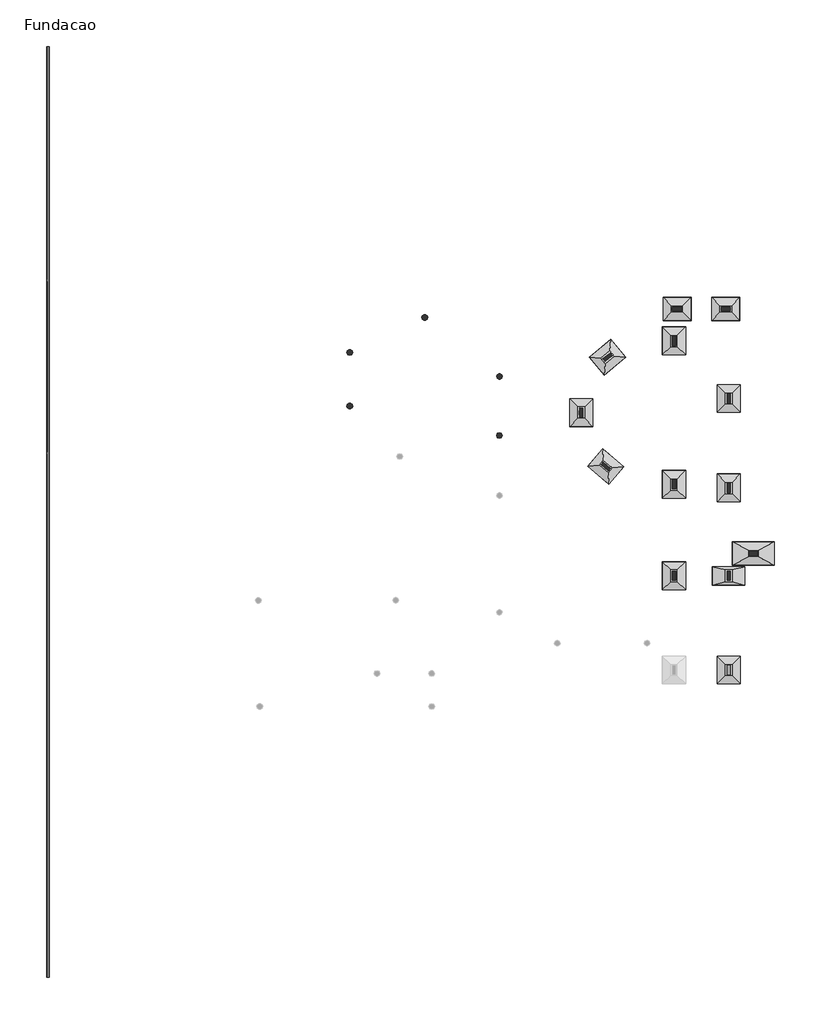
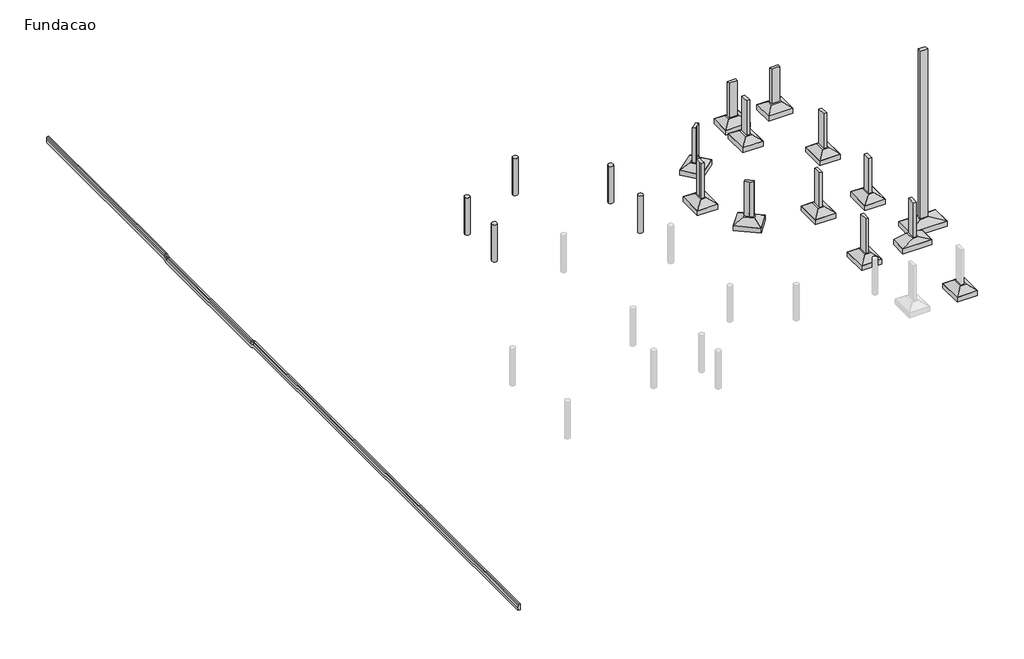
# One storey, part 2 of 2: 17 columns, 13 fasteners, 1 proxy.
# Revit data of these elements (continued)
# Element 3 (IfcColumn, "TQS - Pilar circular : TQS - Pilar circular 25.0cm") (continued)
#   Concreto C = ""
#   Taxa de armadura (kgf/m³) = 0
#   Carga (tf/m²) = 0
#   Carga (tf/m) = 0
#   Carga (tf) = 0
#   Altura = 1.70 m
#   Rebaixo = 0.00 m
#   Altura da fundacao = 0.00 m
#   Largura = 0.00 m
#   Distancia a face = 0.00 m
#   Distancia ao eixo = 0.00 m
#   Resultado de Ensaios fck (MPa) = 0
#   Unique TQS ID = -767
#   Principal = yes
#   Nasce = yes
#   Morre = yes
#   Cabeca de Pilar = no
#   Structural Material = Concrete - Cast-in-Place Concrete
#   Phase Created = CC_AP/ESTR
#   Materials on its faces: "Concrete - Cast-in-Place Concrete"
# Element 4 (IfcColumn, "TQS - Pilar circular : TQS - Pilar circular 25.0cm")
#   Uso = "ESTRUTURA"
#   Titulo = "B3"
#   Chave = "B3//0"
#   Tipo Elemento = "Pilar"
#   SHA1 = "B4824BA6EB04DBA88013BAD919A11F987E93A8CE"
#   Revisão = ""
#   Tipo de carga = ""
#   Divisor de flexao = ""
#   Secao = "C 25"
#   Configuracao = ""
#   Angulo (graus) = ""
#   Detalhamento = ""
#   Casos de vento manual = ""
#   Tipo = ""
#   Alcas = ""
#   Furos = ""
#   Pino = ""
#   Distribuicao = ""
#   Solidarizado = ""
#   Solidarizar na montagem = ""
#   Unir com o próximo = ""
#   Grupo pre moldado = ""
#   Verificado = ""
#   Concreto C = ""
#   Taxa de armadura (kgf/m³) = 0
#   Carga (tf/m²) = 0
#   Carga (tf/m) = 0
#   Carga (tf) = 0
#   Altura = 1.70 m
#   Rebaixo = 0.00 m
#   Altura da fundacao = 0.00 m
#   Largura = 0.00 m
#   Distancia a face = 0.00 m
#   Distancia ao eixo = 0.00 m
#   Resultado de Ensaios fck (MPa) = 0
#   Unique TQS ID = -768
#   Principal = yes
#   Nasce = yes
#   Morre = yes
#   Cabeca de Pilar = no
#   Structural Material = Concrete - Cast-in-Place Concrete
#   Phase Created = CC_AP/ESTR
#   Materials on its faces: "Concrete - Cast-in-Place Concrete"
# Element 5 (IfcColumn, "TQS - Pilar circular : TQS - Pilar circular 25.0cm")
#   Uso = "ESTRUTURA"
#   Titulo = "B2"
#   Chave = "B2//0"
#   Tipo Elemento = "Pilar"
#   SHA1 = "4CE2E912DC9B0318D735B89447CA6954BE93FBBD"
#   Revisão = ""
#   Tipo de carga = ""
#   Divisor de flexao = ""
#   Secao = "C 25"
#   Configuracao = ""
#   Angulo (graus) = ""
#   Detalhamento = ""
#   Casos de vento manual = ""
#   Tipo = ""
#   Alcas = ""
#   Furos = ""
#   Pino = ""
#   Distribuicao = ""
#   Solidarizado = ""
#   Solidarizar na montagem = ""
#   Unir com o próximo = ""
#   Grupo pre moldado = ""
#   Verificado = ""
#   Concreto C = ""
#   Taxa de armadura (kgf/m³) = 0
#   Carga (tf/m²) = 0
#   Carga (tf/m) = 0
#   Carga (tf) = 0
#   Altura = 1.70 m
#   Rebaixo = 0.00 m
#   Altura da fundacao = 0.00 m
#   Largura = 0.00 m
#   Distancia a face = 0.00 m
#   Distancia ao eixo = 0.00 m
#   Resultado de Ensaios fck (MPa) = 0
#   Unique TQS ID = -773
#   Principal = yes
#   Nasce = yes
#   Morre = yes
#   Cabeca de Pilar = no
#   Structural Material = Concrete - Cast-in-Place Concrete
#   Phase Created = CC_AP/ESTR
#   Materials on its faces: "Concrete - Cast-in-Place Concrete"
# Element 6 (IfcColumn, "TQS - Pilar circular : TQS - Pilar circular 25.0cm")
#   Uso = "ESTRUTURA"
#   Titulo = "B4"
#   Chave = "B4//0"
#   Tipo Elemento = "Pilar"
#   SHA1 = "33C063B82A35DA14032FDD3FDBBCC7600ACCE04D"
#   Revisão = ""
#   Tipo de carga = ""
#   Divisor de flexao = ""
#   Secao = "C 25"
#   Configuracao = ""
#   Angulo (graus) = ""
#   Detalhamento = ""
#   Casos de vento manual = ""
#   Tipo = ""
#   Alcas = ""
#   Furos = ""
#   Pino = ""
#   Distribuicao = ""
#   Solidarizado = ""
#   Solidarizar na montagem = ""
#   Unir com o próximo = ""
#   Grupo pre moldado = ""
#   Verificado = ""
#   Concreto C = ""
#   Taxa de armadura (kgf/m³) = 0
#   Carga (tf/m²) = 0
#   Carga (tf/m) = 0
#   Carga (tf) = 0
#   Altura = 1.70 m
#   Rebaixo = 0.00 m
#   Altura da fundacao = 0.00 m
#   Largura = 0.00 m
#   Distancia a face = 0.00 m
#   Distancia ao eixo = 0.00 m
#   Resultado de Ensaios fck (MPa) = 0
#   Unique TQS ID = -774
#   Principal = yes
#   Nasce = yes
#   Morre = yes
#   Cabeca de Pilar = no
#   Structural Material = Concrete - Cast-in-Place Concrete
#   Phase Created = CC_AP/ESTR
#   Materials on its faces: "Concrete - Cast-in-Place Concrete"
# Element 7 (IfcColumn, "TQS - Pilar retangular : 14.0 x 40.0")
#   Uso = "ESTRUTURA"
#   Titulo = "PS1"
#   Chave = "PS1//0"
#   Tipo Elemento = "Pilar"
#   SHA1 = "4597F8CE5B5008DD3216867DEF2D1334C590FC15"
#   Revisão = ""
#   Tipo de carga = ""
#   Divisor de flexao = ""
#   Secao = "R 14/40 270°"
#   Configuracao = ""
#   Angulo (graus) = ""
#   Detalhamento = ""
#   Casos de vento manual = ""
#   Tipo = ""
#   Alcas = ""
#   Furos = ""
#   Pino = ""
#   Distribuicao = ""
#   Solidarizado = ""
#   Solidarizar na montagem = ""
#   Unir com o próximo = ""
#   Grupo pre moldado = ""
#   Verificado = ""
#   Concreto C = ""
#   Taxa de armadura (kgf/m³) = 0
#   Carga (tf/m²) = 0
#   Carga (tf/m) = 0
#   Carga (tf) = 0
#   Altura = 1.70 m
#   Rebaixo = 0.00 m
#   Altura da fundacao = 0.00 m
#   Largura = 0.00 m
#   Distancia a face = 0.00 m
#   Distancia ao eixo = 0.00 m
#   Resultado de Ensaios fck (MPa) = 0
#   Unique TQS ID = -958
#   Principal = yes
#   Nasce = yes
#   Morre = yes
#   Cabeca de Pilar = no
#   Structural Material = Concrete - Cast-in-Place Concrete
#   Phase Created = CC_AP/ESTR
#   Materials on its faces: "Concrete - Cast-in-Place Concrete"
# Element 8 (IfcColumn, "TQS - Pilar retangular : 14.0 x 40.0")
#   Uso = "ESTRUTURA"
#   Titulo = "PS2"
#   Chave = "PS2//0"
#   Tipo Elemento = "Pilar"
#   SHA1 = "1729CD9DA72122FACD843418D908847D3B1966CD"
#   Revisão = ""
#   Tipo de carga = ""
#   Divisor de flexao = ""
#   Secao = "R 14/40 270°"
#   Configuracao = ""
#   Angulo (graus) = ""
#   Detalhamento = ""
#   Casos de vento manual = ""
#   Tipo = ""
#   Alcas = ""
#   Furos = ""
#   Pino = ""
#   Distribuicao = ""
#   Solidarizado = ""
#   Solidarizar na montagem = ""
#   Unir com o próximo = ""
#   Grupo pre moldado = ""
#   Verificado = ""
#   Concreto C = ""
#   Taxa de armadura (kgf/m³) = 0
#   Carga (tf/m²) = 0
#   Carga (tf/m) = 0
#   Carga (tf) = 0
#   Altura = 1.70 m
#   Rebaixo = 0.00 m
#   Altura da fundacao = 0.00 m
#   Largura = 0.00 m
#   Distancia a face = 0.00 m
#   Distancia ao eixo = 0.00 m
#   Resultado de Ensaios fck (MPa) = 0
#   Unique TQS ID = -959
#   Principal = yes
#   Nasce = yes
#   Morre = yes
#   Cabeca de Pilar = no
#   Structural Material = Concrete - Cast-in-Place Concrete
#   Phase Created = CC_AP/ESTR
#   Materials on its faces: "Concrete - Cast-in-Place Concrete"
# Element 9 (IfcColumn, "TQS - Pilar retangular : 14.0 x 40.0")
#   Uso = "ESTRUTURA"
#   Titulo = "PS3"
#   Chave = "PS3//0"
#   Tipo Elemento = "Pilar"
#   SHA1 = "E1C4E1DD2B85E2F78CE9D8770BC24705A0EC4463"
#   Revisão = ""
#   Tipo de carga = ""
#   Divisor de flexao = ""
#   Secao = "R 14/40 180°"
#   Configuracao = ""
#   Angulo (graus) = ""
#   Detalhamento = ""
#   Casos de vento manual = ""
#   Tipo = ""
#   Alcas = ""
#   Furos = ""
#   Pino = ""
#   Distribuicao = ""
#   Solidarizado = ""
#   Solidarizar na montagem = ""
#   Unir com o próximo = ""
#   Grupo pre moldado = ""
#   Verificado = ""
#   Concreto C = ""
#   Taxa de armadura (kgf/m³) = 0
#   Carga (tf/m²) = 0
#   Carga (tf/m) = 0
#   Carga (tf) = 0
#   Altura = 1.70 m
#   Rebaixo = 0.00 m
#   Altura da fundacao = 0.00 m
#   Largura = 0.00 m
#   Distancia a face = 0.00 m
#   Distancia ao eixo = 0.00 m
#   Resultado de Ensaios fck (MPa) = 0
#   Unique TQS ID = -960
#   Principal = yes
#   Nasce = yes
#   Morre = yes
#   Cabeca de Pilar = no
#   Structural Material = Concrete - Cast-in-Place Concrete
#   Phase Created = CC_AP/ESTR
#   Materials on its faces: "Concrete - Cast-in-Place Concrete"
# Element 10 (IfcColumn, "TQS - Pilar retangular : 14.0 x 40.0")
#   Uso = "ESTRUTURA"
#   Titulo = "PS7"
#   Chave = "PS7//0"
#   Tipo Elemento = "Pilar"
#   SHA1 = "EE51B7F018C373FE9CEF53A9864C8051348A9FB9"
#   Revisão = ""
#   Tipo de carga = ""
#   Divisor de flexao = ""
#   Secao = "R 14/40 180°"
#   Configuracao = ""
#   Angulo (graus) = ""
#   Detalhamento = ""
#   Casos de vento manual = ""
#   Tipo = ""
#   Alcas = ""
#   Furos = ""
#   Pino = ""
#   Distribuicao = ""
#   Solidarizado = ""
#   Solidarizar na montagem = ""
#   Unir com o próximo = ""
#   Grupo pre moldado = ""
#   Verificado = ""
#   Concreto C = ""
#   Taxa de armadura (kgf/m³) = 0
#   Carga (tf/m²) = 0
#   Carga (tf/m) = 0
#   Carga (tf) = 0
#   Altura = 1.70 m
#   Rebaixo = 0.00 m
#   Altura da fundacao = 0.00 m
#   Largura = 0.00 m
#   Distancia a face = 0.00 m
#   Distancia ao eixo = 0.00 m
#   Resultado de Ensaios fck (MPa) = 0
#   Unique TQS ID = -964
#   Principal = yes
#   Nasce = yes
#   Morre = yes
#   Cabeca de Pilar = no
#   Structural Material = Concrete - Cast-in-Place Concrete
#   Phase Created = CC_AP/ESTR
#   Materials on its faces: "Concrete - Cast-in-Place Concrete"
# Element 11 (IfcColumn, "TQS - Pilar retangular : 14.0 x 40.0")
#   Uso = "ESTRUTURA"
#   Titulo = "PS8"
#   Chave = "PS8//0"
#   Tipo Elemento = "Pilar"
#   SHA1 = "B515A8CC25CBD0A114828B82A1075E16319BC015"
#   Revisão = ""
#   Tipo de carga = ""
#   Divisor de flexao = ""
#   Secao = "R 14/40 180°"
#   Configuracao = ""
#   Angulo (graus) = ""
#   Detalhamento = ""
#   Casos de vento manual = ""
#   Tipo = ""
#   Alcas = ""
#   Furos = ""
#   Pino = ""
#   Distribuicao = ""
#   Solidarizado = ""
#   Solidarizar na montagem = ""
#   Unir com o próximo = ""
#   Grupo pre moldado = ""
#   Verificado = ""
#   Concreto C = ""
#   Taxa de armadura (kgf/m³) = 0
#   Carga (tf/m²) = 0
#   Carga (tf/m) = 0
#   Carga (tf) = 0
#   Altura = 1.70 m
#   Rebaixo = 0.00 m
#   Altura da fundacao = 0.00 m
#   Largura = 0.00 m
#   Distancia a face = 0.00 m
#   Distancia ao eixo = 0.00 m
#   Resultado de Ensaios fck (MPa) = 0
#   Unique TQS ID = -965
#   Principal = yes
#   Nasce = yes
#   Morre = yes
#   Cabeca de Pilar = no
#   Structural Material = Concrete - Cast-in-Place Concrete
#   Phase Created = CC_AP/ESTR
#   Materials on its faces: "Concrete - Cast-in-Place Concrete"
# Element 12 (IfcColumn, "TQS - Pilar retangular : 14.0 x 40.0")
#   Uso = "ESTRUTURA"
#   Titulo = "PS11"
#   Chave = "PS11//0"
#   Tipo Elemento = "Pilar"
#   SHA1 = "38C3E9E25C80C043D595FE86FE1A911FDC38D350"
#   Revisão = ""
#   Tipo de carga = ""
#   Divisor de flexao = ""
#   Secao = "R 14/40 180°"
#   Configuracao = ""
#   Angulo (graus) = ""
#   Detalhamento = ""
#   Casos de vento manual = ""
#   Tipo = ""
#   Alcas = ""
#   Furos = ""
#   Pino = ""
#   Distribuicao = ""
#   Solidarizado = ""
#   Solidarizar na montagem = ""
#   Unir com o próximo = ""
#   Grupo pre moldado = ""
#   Verificado = ""
#   Concreto C = ""
#   Taxa de armadura (kgf/m³) = 0
#   Carga (tf/m²) = 0
#   Carga (tf/m) = 0
#   Carga (tf) = 0
#   Altura = 1.70 m
#   Rebaixo = 0.00 m
#   Altura da fundacao = 0.00 m
#   Largura = 0.00 m
#   Distancia a face = 0.00 m
#   Distancia ao eixo = 0.00 m
#   Resultado de Ensaios fck (MPa) = 0
#   Unique TQS ID = -968
#   Principal = yes
#   Nasce = yes
#   Morre = yes
#   Cabeca de Pilar = no
#   Structural Material = Concrete - Cast-in-Place Concrete
#   Phase Created = CC_AP/ESTR
#   Materials on its faces: "Concrete - Cast-in-Place Concrete"
# Element 13 (IfcColumn, "TQS - Pilar retangular : 14.0 x 40.0")
#   Uso = "ESTRUTURA"
#   Titulo = "PS12"
#   Chave = "PS12//0"
#   Tipo Elemento = "Pilar"
#   SHA1 = "512D0DE7DB718BC0FE0AECE12A9FB23F7FBE26A9"
#   Revisão = ""
#   Tipo de carga = ""
#   Divisor de flexao = ""
#   Secao = "R 14/40 180°"
#   Configuracao = ""
#   Angulo (graus) = ""
#   Detalhamento = ""
#   Casos de vento manual = ""
#   Tipo = ""
#   Alcas = ""
#   Furos = ""
#   Pino = ""
#   Distribuicao = ""
#   Solidarizado = ""
#   Solidarizar na montagem = ""
#   Unir com o próximo = ""
#   Grupo pre moldado = ""
#   Verificado = ""
#   Concreto C = ""
#   Taxa de armadura (kgf/m³) = 0
#   Carga (tf/m²) = 0
#   Carga (tf/m) = 0
#   Carga (tf) = 0
#   Altura = 1.70 m
#   Rebaixo = 0.00 m
#   Altura da fundacao = 0.00 m
#   Largura = 0.00 m
#   Distancia a face = 0.00 m
#   Distancia ao eixo = 0.00 m
#   Resultado de Ensaios fck (MPa) = 0
#   Unique TQS ID = -969
#   Principal = yes
#   Nasce = yes
#   Morre = yes
#   Cabeca de Pilar = no
#   Structural Material = Concrete - Cast-in-Place Concrete
#   Phase Created = CC_AP/ESTR
#   Materials on its faces: "Concrete - Cast-in-Place Concrete"
# Element 14 (IfcColumn, "TQS - Pilar retangular : 14.0 x 40.0")
#   Uso = "ESTRUTURA"
#   Titulo = "PS13"
#   Chave = "PS13//0"
#   Tipo Elemento = "Pilar"
#   SHA1 = "8EC8E2C6B90DD4DF760F1D4ED431316ED84D10F2"
#   Revisão = ""
#   Tipo de carga = ""
#   Divisor de flexao = ""
#   Secao = "R 14/40 180°"
#   Configuracao = ""
#   Angulo (graus) = ""
#   Detalhamento = ""
#   Casos de vento manual = ""
#   Tipo = ""
#   Alcas = ""
#   Furos = ""
#   Pino = ""
#   Distribuicao = ""
#   Solidarizado = ""
#   Solidarizar na montagem = ""
#   Unir com o próximo = ""
#   Grupo pre moldado = ""
#   Verificado = ""
#   Concreto C = ""
#   Taxa de armadura (kgf/m³) = 0
#   Carga (tf/m²) = 0
#   Carga (tf/m) = 0
#   Carga (tf) = 0
#   Altura = 1.70 m
#   Rebaixo = 0.00 m
#   Altura da fundacao = 0.00 m
#   Largura = 0.00 m
#   Distancia a face = 0.00 m
#   Distancia ao eixo = 0.00 m
#   Resultado de Ensaios fck (MPa) = 0
#   Unique TQS ID = -970
#   Principal = yes
#   Nasce = yes
#   Morre = yes
#   Cabeca de Pilar = no
#   Structural Material = Concrete - Cast-in-Place Concrete
#   Phase Created = CC_AP/ESTR
#   Materials on its faces: "Concrete - Cast-in-Place Concrete"
# Element 15 (IfcColumn, "TQS - Pilar retangular : 19.0 x 35.0")
#   Uso = "ESTRUTURA"
#   Titulo = "P14"
#   Chave = "P14//0"
#   Tipo Elemento = "Pilar"
#   SHA1 = "6631C03D899D7914EBA5EACF44BE1498A45C603B"
#   Revisão = ""
#   Tipo de carga = ""
#   Divisor de flexao = ""
#   Secao = "R 19/35 90°"
#   Configuracao = ""
#   Angulo (graus) = ""
#   Detalhamento = ""
#   Casos de vento manual = ""
#   Tipo = ""
#   Alcas = ""
#   Furos = ""
#   Pino = ""
#   Distribuicao = ""
#   Solidarizado = ""
#   Solidarizar na montagem = ""
#   Unir com o próximo = ""
#   Grupo pre moldado = ""
#   Verificado = ""
#   Concreto C = ""
#   Taxa de armadura (kgf/m³) = 0
#   Carga (tf/m²) = 0
#   Carga (tf/m) = 0
#   Carga (tf) = 0
#   Altura = 7.85 m
#   Rebaixo = 0.00 m
#   Altura da fundacao = 0.00 m
#   Largura = 0.00 m
#   Distancia a face = 0.00 m
#   Distancia ao eixo = 0.00 m
#   Resultado de Ensaios fck (MPa) = 0
#   Unique TQS ID = -30
#   Principal = yes
#   Nasce = yes
#   Morre = yes
#   Cabeca de Pilar = no
#   Structural Material = Concrete - Cast-in-Place Concrete
#   Phase Created = CC_AP/ESTR
#   Materials on its faces: "Concrete - Cast-in-Place Concrete"
# Element 16 (IfcColumn, "TQS - Pilar Polig_1 : TQS Column")
#   Uso = "ESTRUTURA"
#   Titulo = "PS4"
#   Chave = "PS4//0"
#   Tipo Elemento = "Pilar"
#   SHA1 = "CAF5758E71A5FE097847EBD6542E0EE23CE53B7B"
#   Revisão = ""
#   Tipo de carga = ""
#   Divisor de flexao = ""
#   Secao = "P  - Poligonal"
#   Configuracao = ""
#   Angulo (graus) = ""
#   Detalhamento = ""
#   Casos de vento manual = ""
#   Tipo = ""
#   Alcas = ""
#   Furos = ""
#   Pino = ""
#   Distribuicao = ""
#   Solidarizado = ""
#   Solidarizar na montagem = ""
#   Unir com o próximo = ""
#   Grupo pre moldado = ""
#   Verificado = ""
#   Concreto C = ""
#   Taxa de armadura (kgf/m³) = 0
#   Carga (tf/m²) = 0
#   Carga (tf/m) = 0
#   Carga (tf) = 0
#   Altura = 1.70 m
#   Rebaixo = 0.00 m
#   Altura da fundacao = 0.00 m
#   Largura = 0.00 m
#   Distancia a face = 0.00 m
#   Distancia ao eixo = 0.00 m
#   Resultado de Ensaios fck (MPa) = 0
#   Unique TQS ID = -961
#   Principal = yes
#   Nasce = yes
#   Morre = yes
#   Cabeca de Pilar = no
#   Structural Material = Concrete - Cast-in-Place Concrete
#   Phase Created = CC_AP/ESTR
# Element 17 (IfcColumn, "TQS - Pilar Polig_1 : TQS Column")
#   Uso = "ESTRUTURA"
#   Titulo = "PS5"
#   Chave = "PS5//0"
#   Tipo Elemento = "Pilar"
#   SHA1 = "AE9BDBDC0B1786B9555B7E0CE4AAD4E849800AD1"
#   Revisão = ""
#   Tipo de carga = ""
#   Divisor de flexao = ""
#   Secao = "P  - Poligonal"
#   Configuracao = ""
#   Angulo (graus) = ""
#   Detalhamento = ""
#   Casos de vento manual = ""
#   Tipo = ""
#   Alcas = ""
#   Furos = ""
#   Pino = ""
#   Distribuicao = ""
#   Solidarizado = ""
#   Solidarizar na montagem = ""
#   Unir com o próximo = ""
#   Grupo pre moldado = ""
#   Verificado = ""
#   Concreto C = ""
#   Taxa de armadura (kgf/m³) = 0
#   Carga (tf/m²) = 0
#   Carga (tf/m) = 0
#   Carga (tf) = 0
#   Altura = 1.70 m
#   Rebaixo = 0.00 m
#   Altura da fundacao = 0.00 m
#   Largura = 0.00 m
#   Distancia a face = 0.00 m
#   Distancia ao eixo = 0.00 m
#   Resultado de Ensaios fck (MPa) = 0
#   Unique TQS ID = -962
#   Principal = yes
#   Nasce = yes
#   Morre = yes
#   Cabeca de Pilar = no
#   Structural Material = Concrete - Cast-in-Place Concrete
#   Phase Created = CC_AP/ESTR
# Element 18 (IfcColumn, "TQS - Pilar Polig_2 : TQS Column")
#   Uso = "ESTRUTURA"
#   Titulo = "PS6"
#   Chave = "PS6//0"
#   Tipo Elemento = "Pilar"
#   SHA1 = "07EEAEB0E5A3D9C7C5812BCB6FDA506A68E4D4F2"
#   Revisão = ""
#   Tipo de carga = ""
#   Divisor de flexao = ""
#   Secao = "P  - Poligonal"
#   Configuracao = ""
#   Angulo (graus) = ""
#   Detalhamento = ""
#   Casos de vento manual = ""
#   Tipo = ""
#   Alcas = ""
#   Furos = ""
#   Pino = ""
#   Distribuicao = ""
#   Solidarizado = ""
#   Solidarizar na montagem = ""
#   Unir com o próximo = ""
#   Grupo pre moldado = ""
#   Verificado = ""
#   Concreto C = ""
#   Taxa de armadura (kgf/m³) = 0
#   Carga (tf/m²) = 0
#   Carga (tf/m) = 0
#   Carga (tf) = 0
#   Altura = 1.70 m
#   Rebaixo = 0.00 m
#   Altura da fundacao = 0.00 m
#   Largura = 0.00 m
#   Distancia a face = 0.00 m
#   Distancia ao eixo = 0.00 m
#   Resultado de Ensaios fck (MPa) = 0
#   Unique TQS ID = -963
#   Principal = yes
#   Nasce = yes
#   Morre = yes
#   Cabeca de Pilar = no
#   Structural Material = Concrete - Cast-in-Place Concrete
#   Phase Created = CC_AP/ESTR
# Element 19 (IfcFastener, "TQS - Sapata : S14")
#   Uso = "ESTRUTURA"
#   Titulo = "S14"
#   Chave = "-1550"
#   Tipo Elemento = "Fundação"
#   SHA1 = "1357E856F80250D7EFC9EC1E050D5963CC884844"
#   Revisão = ""
#   Tipo de carga = ""
#   Divisor de flexao = ""
#   Secao = ""
#   Configuracao = ""
#   Angulo (graus) = ""
#   Detalhamento = ""
#   Casos de vento manual = ""
#   Tipo = "Sapata"
#   Dimensoes = "100.0,180.0"
#   Estacas = ""
#   Calice = ""
#   Rugosidade = ""
#   Alcas = ""
#   Furos = ""
#   Pino = ""
#   Distribuicao = ""
#   Solidarizado = ""
#   Solidarizar na montagem = ""
#   Unir com o próximo = ""
#   Grupo pre moldado = ""
#   Verificado = ""
#   Concreto C = ""
#   Taxa de armadura (kgf/m³) = 0
#   Carga (tf/m²) = 0
#   Carga (tf/m) = 0
#   Carga (tf) = 0
#   Altura = 0.00 m
#   Rebaixo = 0.00 m
#   Pilar ficticio = 0.00 m
#   Topo = -1.45 m
#   Altura total = 0.50 m
#   Rodape = 0.00 m
#   Diametro = 0.00 m
#   Altura dentro do bloco = 0.00 m
#   Entre eixos = 0.00 m
#   Paredes = 0.00 m
#   Caimento = 0.00 m
#   Largura = 0.00 m
#   Distancia a face = 0.00 m
#   Distancia ao eixo = 0.00 m
#   Resultado de Ensaios fck (MPa) = 0
#   Unique TQS ID = -1550
#   Principal = yes
#   Phase Created = CC_AP/ESTR
#   Materials on its faces: "Concreto - Concreto concretado no local"
# Element 20 (IfcFastener, "TQS - Sapata : SPS1")
#   Uso = "ESTRUTURA"
#   Titulo = "SPS1"
#   Chave = "-1512"
#   Tipo Elemento = "Fundação"
#   SHA1 = "0DB0C78ACFE2E409544A77F7853F60381CB93818"
#   Revisão = ""
#   Tipo de carga = ""
#   Divisor de flexao = ""
#   Secao = ""
#   Configuracao = ""
#   Angulo (graus) = ""
#   Detalhamento = ""
#   Casos de vento manual = ""
#   Tipo = "Sapata"
#   Dimensoes = "100.0,120.0"
#   Estacas = ""
#   Calice = ""
#   Rugosidade = ""
#   Alcas = ""
#   Furos = ""
#   Pino = ""
#   Distribuicao = ""
#   Solidarizado = ""
#   Solidarizar na montagem = ""
#   Unir com o próximo = ""
#   Grupo pre moldado = ""
#   Verificado = ""
#   Concreto C = ""
#   Taxa de armadura (kgf/m³) = 0
#   Carga (tf/m²) = 0
#   Carga (tf/m) = 0
#   Carga (tf) = 0
#   Altura = 0.00 m
#   Rebaixo = 0.00 m
#   Pilar ficticio = 0.00 m
#   Topo = -1.45 m
#   Altura total = 0.50 m
#   Rodape = 0.00 m
#   Diametro = 0.00 m
#   Altura dentro do bloco = 0.00 m
#   Entre eixos = 0.00 m
#   Paredes = 0.00 m
#   Caimento = 0.00 m
#   Largura = 0.00 m
#   Distancia a face = 0.00 m
#   Distancia ao eixo = 0.00 m
#   Resultado de Ensaios fck (MPa) = 0
#   Unique TQS ID = -1512
#   Principal = yes
#   Phase Created = CC_AP/ESTR
#   Materials on its faces: "Concreto - Concreto concretado no local"
# Element 21 (IfcFastener, "TQS - Sapata : SPS10")
#   Uso = "ESTRUTURA"
#   Titulo = "SPS10"
#   Chave = "-1543"
#   Tipo Elemento = "Fundação"
#   SHA1 = "612F949682BC8906AE43999ACE3B00A4C616A0A8"
#   Revisão = ""
#   Tipo de carga = ""
#   Divisor de flexao = ""
#   Secao = ""
#   Configuracao = ""
#   Angulo (graus) = ""
#   Detalhamento = ""
#   Casos de vento manual = ""
#   Tipo = "Sapata"
#   Dimensoes = "100.0,120.0"
#   Estacas = ""
#   Calice = ""
#   Rugosidade = ""
#   Alcas = ""
#   Furos = ""
#   Pino = ""
#   Distribuicao = ""
#   Solidarizado = ""
#   Solidarizar na montagem = ""
#   Unir com o próximo = ""
#   Grupo pre moldado = ""
#   Verificado = ""
#   Concreto C = ""
#   Taxa de armadura (kgf/m³) = 0
#   Carga (tf/m²) = 0
#   Carga (tf/m) = 0
#   Carga (tf) = 0
#   Altura = 0.00 m
#   Rebaixo = 0.00 m
#   Pilar ficticio = 0.00 m
#   Topo = -1.45 m
#   Altura total = 0.50 m
#   Rodape = 0.00 m
#   Diametro = 0.00 m
#   Altura dentro do bloco = 0.00 m
#   Entre eixos = 0.00 m
#   Paredes = 0.00 m
#   Caimento = 0.00 m
#   Largura = 0.00 m
#   Distancia a face = 0.00 m
#   Distancia ao eixo = 0.00 m
#   Resultado de Ensaios fck (MPa) = 0
#   Unique TQS ID = -1543
#   Principal = yes
#   Phase Created = CC_AP/ESTR
#   Materials on its faces: "Concreto - Concreto concretado no local"
# Element 22 (IfcFastener, "TQS - Sapata : SPS11")
#   Uso = "ESTRUTURA"
#   Titulo = "SPS11"
#   Chave = "-1544"
#   Tipo Elemento = "Fundação"
#   SHA1 = "678A094029D3186700C53CC9859E21CCB03EEAB8"
#   Revisão = ""
#   Tipo de carga = ""
#   Divisor de flexao = ""
#   Secao = ""
#   Configuracao = ""
#   Angulo (graus) = ""
#   Detalhamento = ""
#   Casos de vento manual = ""
#   Tipo = "Sapata"
#   Dimensoes = "140.0,80.0"
#   Estacas = ""
#   Calice = ""
#   Rugosidade = ""
#   Alcas = ""
#   Furos = ""
#   Pino = ""
#   Distribuicao = ""
#   Solidarizado = ""
#   Solidarizar na montagem = ""
#   Unir com o próximo = ""
#   Grupo pre moldado = ""
#   Verificado = ""
#   Concreto C = ""
#   Taxa de armadura (kgf/m³) = 0
#   Carga (tf/m²) = 0
#   Carga (tf/m) = 0
#   Carga (tf) = 0
#   Altura = 0.00 m
#   Rebaixo = 0.00 m
#   Pilar ficticio = 0.00 m
#   Topo = -1.45 m
#   Altura total = 0.50 m
#   Rodape = 0.00 m
#   Diametro = 0.00 m
#   Altura dentro do bloco = 0.00 m
#   Entre eixos = 0.00 m
#   Paredes = 0.00 m
#   Caimento = 0.00 m
#   Largura = 0.00 m
#   Distancia a face = 0.00 m
#   Distancia ao eixo = 0.00 m
#   Resultado de Ensaios fck (MPa) = 0
#   Unique TQS ID = -1544
#   Principal = yes
#   Phase Created = CC_AP/ESTR
#   Materials on its faces: "Concreto - Concreto concretado no local"
# Element 23 (IfcFastener, "TQS - Sapata : SPS12")
#   Uso = "ESTRUTURA"
#   Titulo = "SPS12"
#   Chave = "-1545"
#   Tipo Elemento = "Fundação"
#   SHA1 = "A892B9C9285BE3407F8B32028442AB264075CE3A"
#   Revisão = ""
#   Tipo de carga = ""
#   Divisor de flexao = ""
#   Secao = ""
#   Configuracao = ""
#   Angulo (graus) = ""
#   Detalhamento = ""
#   Casos de vento manual = ""
#   Tipo = "Sapata"
#   Dimensoes = "100.0,120.0"
#   Estacas = ""
#   Calice = ""
#   Rugosidade = ""
#   Alcas = ""
#   Furos = ""
#   Pino = ""
#   Distribuicao = ""
#   Solidarizado = ""
#   Solidarizar na montagem = ""
#   Unir com o próximo = ""
#   Grupo pre moldado = ""
#   Verificado = ""
#   Concreto C = ""
#   Taxa de armadura (kgf/m³) = 0
#   Carga (tf/m²) = 0
#   Carga (tf/m) = 0
#   Carga (tf) = 0
#   Altura = 0.00 m
#   Rebaixo = 0.00 m
#   Pilar ficticio = 0.00 m
#   Topo = -1.45 m
#   Altura total = 0.50 m
#   Rodape = 0.00 m
#   Diametro = 0.00 m
#   Altura dentro do bloco = 0.00 m
#   Entre eixos = 0.00 m
#   Paredes = 0.00 m
#   Caimento = 0.00 m
#   Largura = 0.00 m
#   Distancia a face = 0.00 m
#   Distancia ao eixo = 0.00 m
#   Resultado de Ensaios fck (MPa) = 0
#   Unique TQS ID = -1545
#   Principal = yes
#   Phase Created = CC_AP/ESTR
#   Materials on its faces: "Concreto - Concreto concretado no local"
# Element 24 (IfcFastener, "TQS - Sapata : SPS13")
#   Uso = "ESTRUTURA"
#   Titulo = "SPS13"
#   Chave = "-1546"
#   Tipo Elemento = "Fundação"
#   SHA1 = "CDD7149D511DCC0D87C76189E976442BBC013FA0"
#   Revisão = ""
#   Tipo de carga = ""
#   Divisor de flexao = ""
#   Secao = ""
#   Configuracao = ""
#   Angulo (graus) = ""
#   Detalhamento = ""
#   Casos de vento manual = ""
#   Tipo = "Sapata"
#   Dimensoes = "100.0,120.0"
#   Estacas = ""
#   Calice = ""
#   Rugosidade = ""
#   Alcas = ""
#   Furos = ""
#   Pino = ""
#   Distribuicao = ""
#   Solidarizado = ""
#   Solidarizar na montagem = ""
#   Unir com o próximo = ""
#   Grupo pre moldado = ""
#   Verificado = ""
#   Concreto C = ""
#   Taxa de armadura (kgf/m³) = 0
#   Carga (tf/m²) = 0
#   Carga (tf/m) = 0
#   Carga (tf) = 0
#   Altura = 0.00 m
#   Rebaixo = 0.00 m
#   Pilar ficticio = 0.00 m
#   Topo = -1.45 m
#   Altura total = 0.50 m
#   Rodape = 0.00 m
#   Diametro = 0.00 m
#   Altura dentro do bloco = 0.00 m
#   Entre eixos = 0.00 m
#   Paredes = 0.00 m
#   Caimento = 0.00 m
#   Largura = 0.00 m
#   Distancia a face = 0.00 m
#   Distancia ao eixo = 0.00 m
#   Resultado de Ensaios fck (MPa) = 0
#   Unique TQS ID = -1546
#   Principal = yes
#   Phase Created = CC_AP/ESTR
#   Materials on its faces: "Concreto - Concreto concretado no local"
# Element 25 (IfcFastener, "TQS - Sapata : SPS2")
#   Uso = "ESTRUTURA"
#   Titulo = "SPS2"
#   Chave = "-1513"
#   Tipo Elemento = "Fundação"
#   SHA1 = "603FADD6DB2EB68781E32AEC81705DC053729A4E"
#   Revisão = ""
#   Tipo de carga = ""
#   Divisor de flexao = ""
#   Secao = ""
#   Configuracao = ""
#   Angulo (graus) = ""
#   Detalhamento = ""
#   Casos de vento manual = ""
#   Tipo = "Sapata"
#   Dimensoes = "100.0,120.0"
#   Estacas = ""
#   Calice = ""
#   Rugosidade = ""
#   Alcas = ""
#   Furos = ""
#   Pino = ""
#   Distribuicao = ""
#   Solidarizado = ""
#   Solidarizar na montagem = ""
#   Unir com o próximo = ""
#   Grupo pre moldado = ""
#   Verificado = ""
#   Concreto C = ""
#   Taxa de armadura (kgf/m³) = 0
#   Carga (tf/m²) = 0
#   Carga (tf/m) = 0
#   Carga (tf) = 0
#   Altura = 0.00 m
#   Rebaixo = 0.00 m
#   Pilar ficticio = 0.00 m
#   Topo = -1.45 m
#   Altura total = 0.50 m
#   Rodape = 0.00 m
#   Diametro = 0.00 m
#   Altura dentro do bloco = 0.00 m
#   Entre eixos = 0.00 m
#   Paredes = 0.00 m
#   Caimento = 0.00 m
#   Largura = 0.00 m
#   Distancia a face = 0.00 m
#   Distancia ao eixo = 0.00 m
#   Resultado de Ensaios fck (MPa) = 0
#   Unique TQS ID = -1513
#   Principal = yes
#   Phase Created = CC_AP/ESTR
#   Materials on its faces: "Concreto - Concreto concretado no local"
# Element 26 (IfcFastener, "TQS - Sapata : SPS3")
#   Uso = "ESTRUTURA"
#   Titulo = "SPS3"
#   Chave = "-1536"
#   Tipo Elemento = "Fundação"
#   SHA1 = "79306587FBF9E385D4E688BE4182F1340258C694"
#   Revisão = ""
#   Tipo de carga = ""
#   Divisor de flexao = ""
#   Secao = ""
#   Configuracao = ""
#   Angulo (graus) = ""
#   Detalhamento = ""
#   Casos de vento manual = ""
#   Tipo = "Sapata"
#   Dimensoes = "100.0,120.0"
#   Estacas = ""
#   Calice = ""
#   Rugosidade = ""
#   Alcas = ""
#   Furos = ""
#   Pino = ""
#   Distribuicao = ""
#   Solidarizado = ""
#   Solidarizar na montagem = ""
#   Unir com o próximo = ""
#   Grupo pre moldado = ""
#   Verificado = ""
#   Concreto C = ""
#   Taxa de armadura (kgf/m³) = 0
#   Carga (tf/m²) = 0
#   Carga (tf/m) = 0
#   Carga (tf) = 0
#   Altura = 0.00 m
#   Rebaixo = 0.00 m
#   Pilar ficticio = 0.00 m
#   Topo = -1.45 m
#   Altura total = 0.50 m
#   Rodape = 0.00 m
#   Diametro = 0.00 m
#   Altura dentro do bloco = 0.00 m
#   Entre eixos = 0.00 m
#   Paredes = 0.00 m
#   Caimento = 0.00 m
#   Largura = 0.00 m
#   Distancia a face = 0.00 m
#   Distancia ao eixo = 0.00 m
#   Resultado de Ensaios fck (MPa) = 0
#   Unique TQS ID = -1536
#   Principal = yes
#   Phase Created = CC_AP/ESTR
#   Materials on its faces: "Concreto - Concreto concretado no local"
# Element 27 (IfcFastener, "TQS - Sapata : SPS4")
#   Uso = "ESTRUTURA"
#   Titulo = "SPS4"
#   Chave = "-1537"
#   Tipo Elemento = "Fundação"
#   SHA1 = "C7F246035C6D677E4D229288FD6DAFF5BD781782"
#   Revisão = ""
#   Tipo de carga = ""
#   Divisor de flexao = ""
#   Secao = ""
#   Configuracao = ""
#   Angulo (graus) = ""
#   Detalhamento = ""
#   Casos de vento manual = ""
#   Tipo = "Sapata"
#   Dimensoes = "100.0,120.0"
#   Estacas = ""
#   Calice = ""
#   Rugosidade = ""
#   Alcas = ""
#   Furos = ""
#   Pino = ""
#   Distribuicao = ""
#   Solidarizado = ""
#   Solidarizar na montagem = ""
#   Unir com o próximo = ""
#   Grupo pre moldado = ""
#   Verificado = ""
#   Concreto C = ""
#   Taxa de armadura (kgf/m³) = 0
#   Carga (tf/m²) = 0
#   Carga (tf/m) = 0
#   Carga (tf) = 0
#   Altura = 0.00 m
#   Rebaixo = 0.00 m
#   Pilar ficticio = 0.00 m
#   Topo = -1.45 m
#   Altura total = 0.50 m
#   Rodape = 0.00 m
#   Diametro = 0.00 m
#   Altura dentro do bloco = 0.00 m
#   Entre eixos = 0.00 m
#   Paredes = 0.00 m
#   Caimento = 0.00 m
#   Largura = 0.00 m
#   Distancia a face = 0.00 m
#   Distancia ao eixo = 0.00 m
#   Resultado de Ensaios fck (MPa) = 0
#   Unique TQS ID = -1537
#   Principal = yes
#   Phase Created = CC_AP/ESTR
#   Materials on its faces: "Concreto - Concreto concretado no local"
# Element 28 (IfcFastener, "TQS - Sapata : SPS5")
#   Uso = "ESTRUTURA"
#   Titulo = "SPS5"
#   Chave = "-1538"
#   Tipo Elemento = "Fundação"
#   SHA1 = "42CB63A1D6FD1F93305BB9397719DE24CD6D6A3F"
#   Revisão = ""
#   Tipo de carga = ""
#   Divisor de flexao = ""
#   Secao = ""
#   Configuracao = ""
#   Angulo (graus) = ""
#   Detalhamento = ""
#   Casos de vento manual = ""
#   Tipo = "Sapata"
#   Dimensoes = "100.0,120.0"
#   Estacas = ""
#   Calice = ""
#   Rugosidade = ""
#   Alcas = ""
#   Furos = ""
#   Pino = ""
#   Distribuicao = ""
#   Solidarizado = ""
#   Solidarizar na montagem = ""
#   Unir com o próximo = ""
#   Grupo pre moldado = ""
#   Verificado = ""
#   Concreto C = ""
#   Taxa de armadura (kgf/m³) = 0
#   Carga (tf/m²) = 0
#   Carga (tf/m) = 0
#   Carga (tf) = 0
#   Altura = 0.00 m
#   Rebaixo = 0.00 m
#   Pilar ficticio = 0.00 m
#   Topo = -1.45 m
#   Altura total = 0.50 m
#   Rodape = 0.00 m
#   Diametro = 0.00 m
#   Altura dentro do bloco = 0.00 m
#   Entre eixos = 0.00 m
#   Paredes = 0.00 m
#   Caimento = 0.00 m
#   Largura = 0.00 m
#   Distancia a face = 0.00 m
#   Distancia ao eixo = 0.00 m
#   Resultado de Ensaios fck (MPa) = 0
#   Unique TQS ID = -1538
#   Principal = yes
#   Phase Created = CC_AP/ESTR
#   Materials on its faces: "Concreto - Concreto concretado no local"
# Element 29 (IfcFastener, "TQS - Sapata : SPS6")
#   Uso = "ESTRUTURA"
#   Titulo = "SPS6"
#   Chave = "-1539"
#   Tipo Elemento = "Fundação"
#   SHA1 = "7089DE54C758E879502D9964BA83D8ECE2A73D29"
#   Revisão = ""
#   Tipo de carga = ""
#   Divisor de flexao = ""
#   Secao = ""
#   Configuracao = ""
#   Angulo (graus) = ""
#   Detalhamento = ""
#   Casos de vento manual = ""
#   Tipo = "Sapata"
#   Dimensoes = "100.0,120.0"
#   Estacas = ""
#   Calice = ""
#   Rugosidade = ""
#   Alcas = ""
#   Furos = ""
#   Pino = ""
#   Distribuicao = ""
#   Solidarizado = ""
#   Solidarizar na montagem = ""
#   Unir com o próximo = ""
#   Grupo pre moldado = ""
#   Verificado = ""
#   Concreto C = ""
#   Taxa de armadura (kgf/m³) = 0
#   Carga (tf/m²) = 0
#   Carga (tf/m) = 0
#   Carga (tf) = 0
#   Altura = 0.00 m
#   Rebaixo = 0.00 m
#   Pilar ficticio = 0.00 m
#   Topo = -1.45 m
#   Altura total = 0.50 m
#   Rodape = 0.00 m
#   Diametro = 0.00 m
#   Altura dentro do bloco = 0.00 m
#   Entre eixos = 0.00 m
#   Paredes = 0.00 m
#   Caimento = 0.00 m
#   Largura = 0.00 m
#   Distancia a face = 0.00 m
#   Distancia ao eixo = 0.00 m
#   Resultado de Ensaios fck (MPa) = 0
#   Unique TQS ID = -1539
#   Principal = yes
#   Phase Created = CC_AP/ESTR
#   Materials on its faces: "Concreto - Concreto concretado no local"
# Element 30 (IfcFastener, "TQS - Sapata : SPS7")
#   Uso = "ESTRUTURA"
#   Titulo = "SPS7"
#   Chave = "-1540"
#   Tipo Elemento = "Fundação"
#   SHA1 = "39B73FB21C78E38761EEBB9B530BC320EF12A224"
#   Revisão = ""
#   Tipo de carga = ""
#   Divisor de flexao = ""
#   Secao = ""
#   Configuracao = ""
#   Angulo (graus) = ""
#   Detalhamento = ""
#   Casos de vento manual = ""
#   Tipo = "Sapata"
#   Dimensoes = "100.0,120.0"
#   Estacas = ""
#   Calice = ""
#   Rugosidade = ""
#   Alcas = ""
#   Furos = ""
#   Pino = ""
#   Distribuicao = ""
#   Solidarizado = ""
#   Solidarizar na montagem = ""
#   Unir com o próximo = ""
#   Grupo pre moldado = ""
#   Verificado = ""
#   Concreto C = ""
#   Taxa de armadura (kgf/m³) = 0
#   Carga (tf/m²) = 0
#   Carga (tf/m) = 0
#   Carga (tf) = 0
#   Altura = 0.00 m
#   Rebaixo = 0.00 m
#   Pilar ficticio = 0.00 m
#   Topo = -1.45 m
#   Altura total = 0.50 m
#   Rodape = 0.00 m
#   Diametro = 0.00 m
#   Altura dentro do bloco = 0.00 m
#   Entre eixos = 0.00 m
#   Paredes = 0.00 m
#   Caimento = 0.00 m
#   Largura = 0.00 m
#   Distancia a face = 0.00 m
#   Distancia ao eixo = 0.00 m
#   Resultado de Ensaios fck (MPa) = 0
#   Unique TQS ID = -1540
#   Principal = yes
#   Phase Created = CC_AP/ESTR
#   Materials on its faces: "Concreto - Concreto concretado no local"
# Element 31 (IfcFastener, "TQS - Sapata : SPS8")
#   Uso = "ESTRUTURA"
#   Titulo = "SPS8"
#   Chave = "-1541"
#   Tipo Elemento = "Fundação"
#   SHA1 = "4A93414E3DCF89A88E00352BDC704547AD7A716D"
#   Revisão = ""
#   Tipo de carga = ""
#   Divisor de flexao = ""
#   Secao = ""
#   Configuracao = ""
#   Angulo (graus) = ""
#   Detalhamento = ""
#   Casos de vento manual = ""
#   Tipo = "Sapata"
#   Dimensoes = "100.0,120.0"
#   Estacas = ""
#   Calice = ""
#   Rugosidade = ""
#   Alcas = ""
#   Furos = ""
#   Pino = ""
#   Distribuicao = ""
#   Solidarizado = ""
#   Solidarizar na montagem = ""
#   Unir com o próximo = ""
#   Grupo pre moldado = ""
#   Verificado = ""
#   Concreto C = ""
#   Taxa de armadura (kgf/m³) = 0
#   Carga (tf/m²) = 0
#   Carga (tf/m) = 0
#   Carga (tf) = 0
#   Altura = 0.00 m
#   Rebaixo = 0.00 m
#   Pilar ficticio = 0.00 m
#   Topo = -1.45 m
#   Altura total = 0.50 m
#   Rodape = 0.00 m
#   Diametro = 0.00 m
#   Altura dentro do bloco = 0.00 m
#   Entre eixos = 0.00 m
#   Paredes = 0.00 m
#   Caimento = 0.00 m
#   Largura = 0.00 m
#   Distancia a face = 0.00 m
#   Distancia ao eixo = 0.00 m
#   Resultado de Ensaios fck (MPa) = 0
#   Unique TQS ID = -1541
#   Principal = yes
#   Phase Created = CC_AP/ESTR
#   Materials on its faces: "Concreto - Concreto concretado no local"
# Materials
#   "Concrete - Cast-in-Place Concrete": class "Unassigned", colour RGB 192 192 192, transparency 0
#   "Concreto - Concreto concretado no local": class "Concreto", colour RGB 192 192 192, transparency 0
#   ".PAVIMENTAÇÃO CALÇADA": class ".CC_PAVIMENTAÇÃO", colour RGB 176 176 176, transparency 0, Description = "Pavimentação calçada cinza claro", Cost = 0
